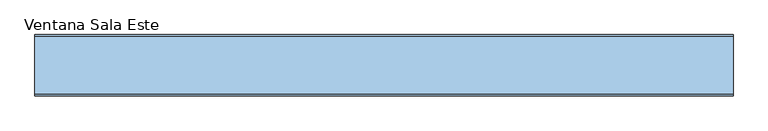
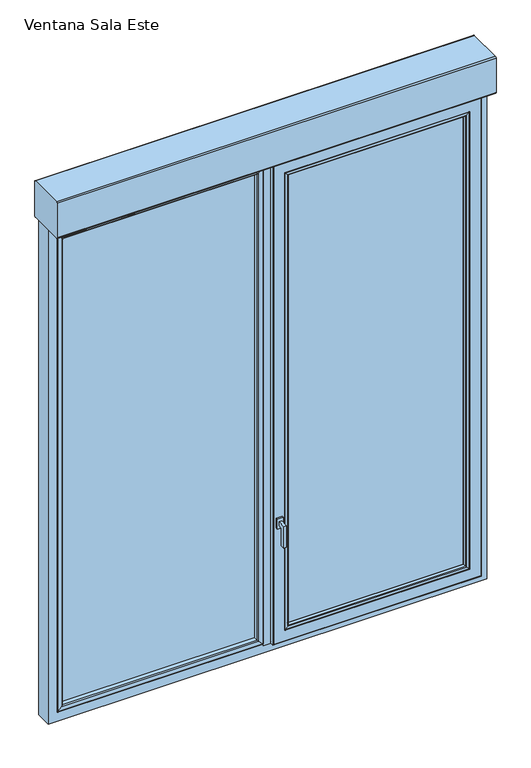
"""IFC4 building model written with IfcOpenShell, lengths in millimetres: window geometry, 2019_ES_Ventana_Replus_re80pvc301_11103_box_1-Hoja_Panel-Fijo-Lateral_con-Compacto : Ventana Sala Este."""

from ifc_helpers import new_model, si_unit, point, frame, frame_2d, origin, place, context, project, spatial, polyline, circle_curve, ellipse_curve, trimmed, segment, composite_curve, outline, extrude, source, transform, mapped, element, save
from ifc_brep_helpers import plane_surface, cylinder_surface, advanced_brep


def ventana_sala_este_de1b01aa(model_context):
    return source(origin(), model_context, "Body", "SolidModel", [
        extrude(outline(composite_curve([segment(polyline([(55.0, 3310.0), (-120.0, 3310.0)]), True, "CONTINUOUS"), segment(trimmed(circle_curve(frame_2d((-120.0, 3315.0)), 5.0), [point((-120.0, 3310.0))], [point((-125.0, 3315.0))], False, "CARTESIAN"), True, "CONTINUOUS"), segment(polyline([(-125.0, 3315.0), (-125.0, 3490.0)]), True, "CONTINUOUS"), segment(trimmed(circle_curve(frame_2d((-120.0, 3490.0)), 5.0), [point((-125.0, 3490.0))], [point((-120.0, 3495.0))], False, "CARTESIAN"), True, "CONTINUOUS"), segment(polyline([(-120.0, 3495.0), (55.0, 3495.0)]), True, "CONTINUOUS"), segment(trimmed(circle_curve(frame_2d((55.0, 3490.0)), 5.0), [point((55.0, 3495.0))], [point((60.0, 3490.0))], False, "CARTESIAN"), True, "CONTINUOUS"), segment(polyline([(60.0, 3490.0), (60.0, 3315.0)]), True, "CONTINUOUS"), segment(trimmed(circle_curve(frame_2d((55.0, 3315.0)), 5.0), [point((60.0, 3315.0))], [point((55.0, 3310.0))], False, "CARTESIAN"), True, "CONTINUOUS")], self_intersect=False)), frame((-1050.0, 0.0, 0.0), z_axis=(1.0, 0.0, 0.0), x_axis=(0.0, 1.0, 0.0)), (0.0, 0.0, 1.0), 2100.0),
        extrude(outline(polyline([(-78.4999991, 1470.0), (-78.4999991, 1450.0), (-98.4999991, 1450.0), (-98.4999991, 1360.0), (-118.4999991, 1360.0), (-118.4999991, 1470.0), (-78.4999991, 1470.0)])), frame((38.5, 0.0, 0.0), z_axis=(1.0, 0.0, 0.0), x_axis=(0.0, 1.0, 0.0)), (0.0, 0.0, 1.0), 12.0),
        extrude(outline(polyline([(58.7312385, -78.4999991), (30.2687615, -78.4999991), (30.2687615, -68.4999991), (58.7312385, -68.4999991), (58.7312385, -78.4999991)])), frame((0.0, 0.0, 1435.217127), z_axis=(0.0, 0.0, 1.0), x_axis=(1.0, 0.0, 0.0)), (0.0, 0.0, 1.0), 49.565746),
        extrude(outline(polyline([(-37.0063666, 11.4999962), (-37.0063666, 7.4999962), (-984.1891471, 7.4999962), (-984.1891471, 11.4999962), (-37.0063666, 11.4999962)])), frame((0.0, 0.0, 875.6108529), z_axis=(0.0, 0.0, 1.0), x_axis=(1.0, 0.0, 0.0)), (0.0, 0.0, 1.0), 2368.7782941),
        extrude(outline(polyline([(-37.0063666, -6.5), (-37.0063666, -10.5), (-984.1891471, -10.5), (-984.1891471, -6.5), (-37.0063666, -6.5)])), frame((0.0, 0.0, 875.6108529), z_axis=(0.0, 0.0, 1.0), x_axis=(1.0, 0.0, 0.0)), (0.0, 0.0, 1.0), 2368.7782941),
        extrude(outline(polyline([(-37.0063666, -24.4999997), (-37.0063666, -28.4999997), (-984.1891471, -28.4999997), (-984.1891471, -24.4999997), (-37.0063666, -24.4999997)])), frame((0.0, 0.0, 875.6108529), z_axis=(0.0, 0.0, 1.0), x_axis=(1.0, 0.0, 0.0)), (0.0, 0.0, 1.0), 2368.7782941),
        advanced_brep(
        [(-22.1502489, -49.9816666, 3264.0497511), (-41.8192398, -49.2838062, 3244.3807602), (-41.8192398, -49.2838062, 875.6192398), (-22.1502489, -49.9816666, 855.9502489), (-46.4697163, -45.5846502, 3239.7302837), (-46.4697163, -45.5846502, 880.2697163), (-984.3807594, -49.2838062, 875.6192398), (-1004.0497503, -49.9816666, 855.9502489), (-21.0, -48.871505, 3265.2), (-21.0, -48.871505, 854.8), (-51.0475336, -28.5000036, 3235.1524664), (-51.0475336, -28.5000036, 884.8475336), (-979.7302829, -45.5846502, 880.2697163), (-43.2922784, -28.5000036, 877.0922784), (-982.9077208, -28.5000036, 877.0922784), (-982.9077208, -28.5000036, 3242.9077216), (-43.2922784, -28.5000036, 3242.9077216), (-975.1524657, -28.5000036, 3235.1524664), (-975.1524657, -28.5000036, 884.8475336), (-35.4855, -36.306782, 3250.7145), (-35.4855, -36.306782, 869.2855), (-35.4855, -39.5069121, 3250.7145), (-35.4855, -39.5069121, 869.2855), (-990.7144993, -36.306782, 869.2855), (-21.0, -39.5069121, 854.8), (-1005.1999993, -39.5069121, 854.8), (-1005.1999993, -39.5069121, 3265.2), (-21.0, -39.5069121, 3265.2), (-990.7144993, -39.5069121, 3250.7145), (-990.7144993, -39.5069121, 869.2855), (-1005.1999993, -48.871505, 854.8), (-984.3807594, -49.2838062, 3244.3807602), (-1004.0497503, -49.9816666, 3264.0497511), (-979.7302829, -45.5846502, 3239.7302837), (-990.7144993, -36.306782, 3250.7145), (-1005.1999993, -48.871505, 3265.2)],
        [
            (0, 1),
            (1, 2),
            (2, 3),
            (3, 0),
            (1, 4, ellipse_curve(frame((-41.6449168, -44.2918491, 3244.5550832), z_axis=(0.7071067811865475, 0.0, -0.7071067811865475), x_axis=(0.7071067811865474, 0.0, 0.7071067811865476)), 7.0639967, 4.995)),
            (4, 5),
            (5, 2, ellipse_curve(frame((-41.6449168, -44.2918491, 875.4449168), z_axis=(0.7071067811865475, 0.0, 0.7071067811865475), x_axis=(-0.7071067811865474, 0.0, 0.7071067811865476)), 7.0639967, 4.995)),
            (2, 6),
            (6, 7),
            (7, 3),
            (8, 0, ellipse_curve(frame((-22.1108601, -48.871505, 3264.0891399), z_axis=(0.7071067811865475, 0.0, -0.7071067811865475), x_axis=(0.7071067811865474, 0.0, 0.7071067811865476)), 1.5709935, 1.1108601)),
            (3, 9, ellipse_curve(frame((-22.1108601, -48.871505, 855.9108601), z_axis=(0.7071067811865475, 0.0, 0.7071067811865475), x_axis=(-0.7071067811865474, 0.0, 0.7071067811865476)), 1.5709935, 1.1108601)),
            (9, 8),
            (4, 10),
            (10, 11),
            (11, 5),
            (5, 12),
            (12, 6, ellipse_curve(frame((-984.5550824, -44.2918491, 875.4449168), z_axis=(0.7071067811865475, 0.0, -0.7071067811865475), x_axis=(0.7071067811865476, 0.0, 0.7071067811865474)), 7.0639967, 4.995)),
            (13, 14),
            (14, 15),
            (15, 16),
            (16, 13),
            (10, 17),
            (17, 18),
            (18, 11),
            (18, 12),
            (16, 19),
            (19, 20),
            (20, 13),
            (19, 21),
            (21, 22),
            (22, 20),
            (20, 23),
            (23, 14),
            (24, 25),
            (25, 26),
            (26, 27),
            (27, 24),
            (21, 28),
            (28, 29),
            (29, 22),
            (29, 23),
            (9, 24),
            (27, 8),
            (9, 30),
            (30, 25),
            (7, 30, ellipse_curve(frame((-1004.0891391, -48.871505, 855.9108601), z_axis=(0.7071067811865475, 0.0, -0.7071067811865475), x_axis=(0.7071067811865476, 0.0, 0.7071067811865474)), 1.5709935, 1.1108601)),
            (6, 31),
            (31, 32),
            (32, 7),
            (12, 33),
            (33, 31, ellipse_curve(frame((-984.5550824, -44.2918491, 3244.5550832), z_axis=(-0.7071067811865475, 0.0, -0.7071067811865475), x_axis=(0.7071067811865474, 0.0, -0.7071067811865476)), 7.0639967, 4.995)),
            (17, 33),
            (23, 34),
            (34, 15),
            (28, 34),
            (30, 35),
            (35, 26),
            (32, 35, ellipse_curve(frame((-1004.0891391, -48.871505, 3264.0891399), z_axis=(-0.7071067811865475, 0.0, -0.7071067811865475), x_axis=(0.7071067811865474, 0.0, -0.7071067811865476)), 1.5709935, 1.1108601)),
            (31, 1),
            (0, 32),
            (33, 4),
            (34, 19),
            (35, 8),
        ],
        [
            plane_surface(frame((-41.8192398, -49.2838062, 3244.3807602), z_axis=(-0.03545791932093311, -0.9993711702652975, 0.0), x_axis=(0.0, 0.0, -1.0))),
            cylinder_surface(frame((-41.6449168, -44.2918491, 3272.2), z_axis=(0.0, 0.0, 1.0), x_axis=(-1.0, 0.0, 0.0)), 4.995),
            plane_surface(frame((-41.8192398, -49.2838062, 875.6192398), z_axis=(0.0, -0.9993711702652976, 0.035457919320929884), x_axis=(-1.0, 0.0, 0.0))),
            cylinder_surface(frame((-22.1108601, -48.871505, 3272.2), z_axis=(0.0, 0.0, 1.0), x_axis=(-1.0, 0.0, 0.0)), 1.1108601),
            plane_surface(frame((-51.0475336, -28.5000036, 3235.1524664), z_axis=(-0.9659258262890619, -0.25881904510254483, 0.0), x_axis=(0.0, 0.0, -1.0))),
            cylinder_surface(frame((-14.0, -44.2918491, 875.4449168), z_axis=(1.0, 0.0, 0.0), x_axis=(0.0, 0.0, 1.0)), 4.995),
            plane_surface(frame((-982.9077208, -28.5000036, 3242.9077216), z_axis=(0.0, 1.0, 0.0), x_axis=(1.0, 0.0, 0.0))),
            plane_surface(frame((-51.0475336, -28.5000036, 884.8475336), z_axis=(0.0, -0.25881904510254794, 0.965925826289061), x_axis=(-1.0, 0.0, 0.0))),
            plane_surface(frame((-35.4855, -36.306782, 3250.7145), z_axis=(0.7071067811865617, 0.7071067811865334, 0.0), x_axis=(0.0, 0.0, -1.0))),
            plane_surface(frame((-35.4855, -39.5069121, 3250.7145), z_axis=(1.0, 0.0, 0.0), x_axis=(0.0, 0.0, -1.0))),
            plane_surface(frame((-35.4855, -36.306782, 869.2855), z_axis=(0.0, 0.7071067811865357, -0.7071067811865593), x_axis=(-1.0, 0.0, 0.0))),
            plane_surface(frame((-1005.1999993, -39.5069121, 3265.2), z_axis=(0.0, 1.0, 0.0), x_axis=(1.0, 0.0, 0.0))),
            plane_surface(frame((-35.4855, -39.5069121, 869.2855), z_axis=(0.0, 0.0, -1.0), x_axis=(-1.0, 0.0, 0.0))),
            plane_surface(frame((-21.0, -46.2002121, 3265.2), z_axis=(1.0, 0.0, 0.0), x_axis=(0.0, 0.0, -1.0))),
            plane_surface(frame((-21.0, -46.2002121, 854.8), z_axis=(0.0, 0.0, -1.0), x_axis=(-1.0, 0.0, 0.0))),
            cylinder_surface(frame((-14.0, -48.871505, 855.9108601), z_axis=(1.0, 0.0, 0.0), x_axis=(0.0, 0.0, 1.0)), 1.1108601),
            plane_surface(frame((-984.3807594, -49.2838062, 875.6192398), z_axis=(0.03545791932092666, -0.9993711702652978, 0.0), x_axis=(0.0, 0.0, 1.0))),
            cylinder_surface(frame((-984.5550824, -44.2918491, 847.8), z_axis=(0.0, 0.0, -1.0), x_axis=(1.0, 0.0, 0.0)), 4.995),
            plane_surface(frame((-975.1524657, -28.5000036, 884.8475336), z_axis=(0.9659258262890602, -0.2588190451025511, 0.0), x_axis=(0.0, 0.0, 1.0))),
            plane_surface(frame((-990.7144993, -36.306782, 869.2855), z_axis=(-0.707106781186557, 0.707106781186538, 0.0), x_axis=(0.0, 0.0, 1.0))),
            plane_surface(frame((-990.7144993, -39.5069121, 869.2855), z_axis=(-1.0, 0.0, 0.0), x_axis=(0.0, 0.0, 1.0))),
            plane_surface(frame((-1005.1999993, -46.2002121, 854.8), z_axis=(-1.0, 0.0, 0.0), x_axis=(0.0, 0.0, 1.0))),
            cylinder_surface(frame((-1004.0891391, -48.871505, 847.8), z_axis=(0.0, 0.0, -1.0), x_axis=(1.0, 0.0, 0.0)), 1.1108601),
            plane_surface(frame((-984.3807594, -49.2838062, 3244.3807602), z_axis=(0.0, -0.9993711702652976, -0.035457919320929884), x_axis=(1.0, 0.0, 0.0))),
            cylinder_surface(frame((-1012.1999993, -44.2918491, 3244.5550832), z_axis=(-1.0, 0.0, 0.0), x_axis=(0.0, 0.0, -1.0)), 4.995),
            plane_surface(frame((-975.1524657, -28.5000036, 3235.1524664), z_axis=(0.0, -0.258819045102548, -0.9659258262890611), x_axis=(1.0, 0.0, 0.0))),
            plane_surface(frame((-990.7144993, -36.306782, 3250.7145), z_axis=(0.0, 0.7071067811865357, 0.7071067811865593), x_axis=(1.0, 0.0, 0.0))),
            plane_surface(frame((-990.7144993, -39.5069121, 3250.7145), z_axis=(0.0, 0.0, 1.0), x_axis=(1.0, 0.0, 0.0))),
            plane_surface(frame((-1005.1999993, -46.2002121, 3265.2), z_axis=(0.0, 0.0, 1.0), x_axis=(1.0, 0.0, 0.0))),
            cylinder_surface(frame((-1012.1999993, -48.871505, 3264.0891399), z_axis=(-1.0, 0.0, 0.0), x_axis=(0.0, 0.0, -1.0)), 1.1108601),
        ],
        [
            (0, [[1, 2, 3, 4]]),
            (1, [[5, 6, 7, -2]]),
            (2, [[-3, 8, 9, 10]]),
            (3, [[11, -4, 12, 13]]),
            (4, [[14, 15, 16, -6]]),
            (5, [[-7, 17, 18, -8]]),
            (6, [[19, 20, 21, 22], [23, 24, 25, -15]]),
            (7, [[-16, -25, 26, -17]]),
            (8, [[27, 28, 29, -22]]),
            (9, [[30, 31, 32, -28]]),
            (10, [[-29, 33, 34, -19]]),
            (11, [[35, 36, 37, 38], [39, 40, 41, -31]]),
            (12, [[-32, -41, 42, -33]]),
            (13, [[-13, 43, -38, 44]]),
            (14, [[-43, 45, 46, -35]]),
            (15, [[-12, -10, 47, -45]]),
            (16, [[-9, 48, 49, 50]]),
            (17, [[-18, 51, 52, -48]]),
            (18, [[-26, -24, 53, -51]]),
            (19, [[-34, 54, 55, -20]]),
            (20, [[-42, -40, 56, -54]]),
            (21, [[-46, 57, 58, -36]]),
            (22, [[-47, -50, 59, -57]]),
            (23, [[-49, 60, -1, 61]]),
            (24, [[-52, 62, -5, -60]]),
            (25, [[-53, -23, -14, -62]]),
            (26, [[-55, 63, -27, -21]]),
            (27, [[-56, -39, -30, -63]]),
            (28, [[-58, 64, -44, -37]]),
            (29, [[-59, -61, -11, -64]]),
        ],
    ),
        extrude(outline(polyline([(3207.0, 947.1999993), (3207.0, 81.0), (912.8, 81.0), (912.8, 947.1999993), (3207.0, 947.1999993)]), holes=[polyline([(920.8, 939.1999993), (920.8, 89.0), (3199.0, 89.0), (3199.0, 939.1999993), (920.8, 939.1999993)])]), frame((0.0, -27.0000002, 0.0), z_axis=(0.0, 1.0, 0.0), x_axis=(0.0, 0.0, 1.0)), (0.0, 0.0, 1.0), 16.0000002),
        extrude(outline(polyline([(3207.0, 947.1999993), (3207.0, 81.0), (912.8, 81.0), (912.8, 947.1999993), (3207.0, 947.1999993)]), holes=[polyline([(920.8, 939.1999993), (920.8, 89.0), (3199.0, 89.0), (3199.0, 939.1999993), (920.8, 939.1999993)])]), frame((0.0, -47.0000002, 0.0), z_axis=(0.0, 1.0, 0.0), x_axis=(0.0, 0.0, 1.0)), (0.0, 0.0, 1.0), 16.0000002),
        extrude(outline(polyline([(3238.3891471, -43.0063666), (3238.3891471, -978.1891471), (881.8608529, -978.1891471), (881.8608529, -43.0063666), (3238.3891471, -43.0063666)]), holes=[polyline([(889.8608529, -51.0063666), (889.8608529, -970.1891471), (3230.3891471, -970.1891471), (3230.3891471, -51.0063666), (889.8608529, -51.0063666)])]), frame((0.0, -24.5, 0.0), z_axis=(0.0, 1.0, 0.0), x_axis=(0.0, 0.0, 1.0)), (0.0, 0.0, 1.0), 14.0),
        extrude(outline(polyline([(3238.3891471, -43.0063666), (3238.3891471, -978.1891471), (881.8608529, -978.1891471), (881.8608529, -43.0063666), (3238.3891471, -43.0063666)]), holes=[polyline([(889.8608529, -51.0063666), (889.8608529, -970.1891471), (3230.3891471, -970.1891471), (3230.3891471, -51.0063666), (889.8608529, -51.0063666)])]), frame((0.0, -6.5, 0.0), z_axis=(0.0, 1.0, 0.0), x_axis=(0.0, 0.0, 1.0)), (0.0, 0.0, 1.0), 14.0),
        advanced_brep(
        [(48.1911809, 11.5, 3240.2), (48.1911809, 11.5, 879.8), (48.1911809, -11.9999991, 879.8), (48.1911809, -11.9999991, 3240.2), (980.1999993, 11.5, 3240.2), (980.1999993, 11.5, 879.8), (88.2020856, 11.5, 919.8109047), (940.1890945, 11.5, 919.8109047), (940.1890945, 11.5, 3200.1890953), (88.2020856, 11.5, 3200.1890953), (980.1999993, -11.9999991, 879.8), (35.1911809, -11.9999991, 3253.2), (993.1999993, -11.9999991, 3253.2), (993.1999993, -11.9999991, 866.8), (35.1911809, -11.9999991, 866.8), (980.1999993, -11.9999991, 3240.2), (35.1911809, -50.0, 866.8), (35.1911809, -50.0, 3253.2), (993.1999993, -50.0, 866.8), (15.1911809, -50.0, 3273.2), (1013.1999993, -50.0, 3273.2), (1013.1999993, -50.0, 846.8), (15.1911809, -50.0, 846.8), (993.1999993, -50.0, 3253.2), (15.1911809, -65.4999991, 3273.2), (15.1911809, -65.4999991, 846.8), (1013.1999993, -65.4999991, 846.8), (18.1911809, -68.4999991, 3270.2), (18.1911809, -68.4999991, 849.8), (1010.1999993, -68.4999991, 849.8), (1010.1999993, -68.4999991, 3270.2), (70.9541209, -68.4999991, 3217.43706), (957.4370593, -68.4999991, 3217.43706), (957.4370593, -68.4999991, 902.56294), (70.9541209, -68.4999991, 902.56294), (72.1911809, -67.2629391, 3216.2), (72.1911809, -67.2629391, 903.8), (956.1999993, -67.2629391, 903.8), (72.7423375, -67.7951848, 3215.6488434), (72.7423375, -67.7951848, 904.3511566), (955.6488427, -67.7951848, 904.3511566), (85.7676831, -67.3403297, 3202.6234978), (85.7676831, -67.3403297, 917.3765022), (942.6234971, -67.3403297, 917.3765022), (89.4917884, -64.3780426, 3198.8993925), (89.4917884, -64.3780426, 921.1006075), (938.8993918, -64.3780426, 921.1006075), (92.8970803, -51.6693201, 3195.4941006), (92.8970803, -51.6693201, 924.5058994), (935.4940999, -51.6693201, 924.5058994), (92.3834932, -51.0000003, 3196.0076877), (92.3834932, -51.0000003, 923.9923123), (936.007687, -51.0000003, 923.9923123), (81.1911809, -51.0000003, 3207.2), (947.1999993, -51.0000003, 3207.2), (947.1999993, -51.0000003, 912.8), (81.1911809, -51.0000003, 912.8), (936.007687, -51.0000003, 3196.0076877), (81.1911809, -56.4999995, 3207.2), (81.1911809, -56.4999995, 912.8), (947.1999993, -56.4999995, 912.8), (69.1911809, -56.4999995, 3219.2), (959.1999993, -56.4999995, 3219.2), (959.1999993, -56.4999995, 900.8), (69.1911809, -56.4999995, 900.8), (947.1999993, -56.4999995, 3207.2), (69.1911809, -25.6153717, 3219.2), (69.1911809, -25.6153717, 900.8), (959.1999993, -25.6153717, 900.8), (66.574961, -6.9999997, 3221.8162199), (66.574961, -6.9999997, 898.1837801), (961.8162192, -6.9999997, 898.1837801), (961.8162192, -6.9999997, 3221.8162199), (87.1911809, -6.9999997, 3201.2), (941.1999993, -6.9999997, 3201.2), (941.1999993, -6.9999997, 918.8), (87.1911809, -6.9999997, 918.8), (87.1911809, -3.0000033, 3201.2), (87.1911809, -3.0000033, 918.8), (941.1999993, -3.0000033, 918.8), (941.1999993, -3.0000033, 3201.2), (93.7172496, -3.0000033, 3194.6739313), (934.6739305, -3.0000033, 3194.6739313), (934.6739305, -3.0000033, 925.3260687), (93.7172496, -3.0000033, 925.3260687), (94.2153834, -2.3508228, 3194.1757976), (94.2153834, -2.3508228, 925.8242024), (934.1757968, -2.3508228, 925.8242024), (91.0998631, 9.2764571, 3197.2913178), (91.0998631, 9.2764571, 922.7086822), (937.2913171, 9.2764571, 922.7086822), (1013.1999993, -65.4999991, 3273.2), (956.1999993, -67.2629391, 3216.2), (955.6488427, -67.7951848, 3215.6488434), (942.6234971, -67.3403297, 3202.6234978), (938.8993918, -64.3780426, 3198.8993925), (935.4940999, -51.6693201, 3195.4941006), (959.1999993, -25.6153717, 3219.2), (934.1757968, -2.3508228, 3194.1757976), (937.2913171, 9.2764571, 3197.2913178)],
        [
            (0, 1),
            (1, 2),
            (2, 3),
            (3, 0),
            (0, 4),
            (4, 5),
            (5, 1),
            (6, 7),
            (7, 8),
            (8, 9),
            (9, 6),
            (5, 10),
            (10, 2),
            (11, 12),
            (12, 13),
            (13, 14),
            (14, 11),
            (10, 15),
            (15, 3),
            (14, 16),
            (16, 17),
            (17, 11),
            (13, 18),
            (18, 16),
            (19, 20),
            (20, 21),
            (21, 22),
            (22, 19),
            (18, 23),
            (23, 17),
            (24, 19),
            (22, 25),
            (25, 24),
            (21, 26),
            (26, 25),
            (27, 24, ellipse_curve(frame((18.1911809, -65.4999991, 3270.2), z_axis=(-0.7071067811865475, 0.0, -0.7071067811865475), x_axis=(-0.7071067811865474, 0.0, 0.7071067811865476)), 4.2426407, 3.0)),
            (25, 28, ellipse_curve(frame((18.1911809, -65.4999991, 849.8), z_axis=(-0.7071067811865475, 0.0, 0.7071067811865475), x_axis=(0.7071067811865474, 0.0, 0.7071067811865476)), 4.2426407, 3.0)),
            (28, 27),
            (26, 29, ellipse_curve(frame((1010.1999993, -65.4999991, 849.8), z_axis=(-0.7071067811865475, 0.0, -0.7071067811865475), x_axis=(-0.7071067811865476, 0.0, 0.7071067811865474)), 4.2426407, 3.0)),
            (29, 28),
            (29, 30),
            (30, 27),
            (31, 32),
            (32, 33),
            (33, 34),
            (34, 31),
            (35, 31, ellipse_curve(frame((70.9541209, -67.2629391, 3217.43706), z_axis=(-0.7071067811865475, 0.0, -0.7071067811865475), x_axis=(-0.7071067811865474, 0.0, 0.7071067811865476)), 1.7494671, 1.23706)),
            (34, 36, ellipse_curve(frame((70.9541209, -67.2629391, 902.56294), z_axis=(-0.7071067811865475, 0.0, 0.7071067811865475), x_axis=(0.7071067811865474, 0.0, 0.7071067811865476)), 1.7494671, 1.23706)),
            (36, 35),
            (33, 37, ellipse_curve(frame((957.4370593, -67.2629391, 902.56294), z_axis=(-0.7071067811865475, 0.0, -0.7071067811865475), x_axis=(-0.7071067811865476, 0.0, 0.7071067811865474)), 1.7494671, 1.23706)),
            (37, 36),
            (38, 35, ellipse_curve(frame((72.7237511, -67.2629391, 3215.6674299), z_axis=(-0.7071067811865475, 0.0, -0.7071067811865475), x_axis=(-0.7071067811865474, 0.0, 0.7071067811865476)), 0.7531679, 0.5325701)),
            (36, 39, ellipse_curve(frame((72.7237511, -67.2629391, 904.3325701), z_axis=(-0.7071067811865475, 0.0, 0.7071067811865475), x_axis=(0.7071067811865474, 0.0, 0.7071067811865476)), 0.7531679, 0.5325701)),
            (39, 38),
            (37, 40, ellipse_curve(frame((955.6674291, -67.2629391, 904.3325701), z_axis=(-0.7071067811865475, 0.0, -0.7071067811865475), x_axis=(-0.7071067811865476, 0.0, 0.7071067811865474)), 0.7531679, 0.5325701)),
            (40, 39),
            (41, 38),
            (39, 42),
            (42, 41),
            (40, 43),
            (43, 42),
            (44, 41, ellipse_curve(frame((85.6280851, -63.3427664, 3202.7630958), z_axis=(-0.7071067811865475, 0.0, -0.7071067811865475), x_axis=(-0.7071067811865474, 0.0, 0.7071067811865476)), 5.6568542, 4.0)),
            (42, 45, ellipse_curve(frame((85.6280851, -63.3427664, 917.2369042), z_axis=(-0.7071067811865475, 0.0, 0.7071067811865475), x_axis=(0.7071067811865474, 0.0, 0.7071067811865476)), 5.6568542, 4.0)),
            (45, 44),
            (43, 46, ellipse_curve(frame((942.7630951, -63.3427664, 917.2369042), z_axis=(-0.7071067811865475, 0.0, -0.7071067811865475), x_axis=(-0.7071067811865476, 0.0, 0.7071067811865474)), 5.6568542, 4.0)),
            (46, 45),
            (47, 44),
            (45, 48),
            (48, 47),
            (46, 49),
            (49, 48),
            (50, 47, ellipse_curve(frame((92.3834932, -51.5317048, 3196.0076877), z_axis=(-0.7071067811865475, 0.0, -0.7071067811865475), x_axis=(-0.7071067811865474, 0.0, 0.7071067811865476)), 0.7519437, 0.5317045)),
            (48, 51, ellipse_curve(frame((92.3834932, -51.5317048, 923.9923123), z_axis=(-0.7071067811865475, 0.0, 0.7071067811865475), x_axis=(0.7071067811865474, 0.0, 0.7071067811865476)), 0.7519437, 0.5317045)),
            (51, 50),
            (49, 52, ellipse_curve(frame((936.007687, -51.5317048, 923.9923123), z_axis=(-0.7071067811865475, 0.0, -0.7071067811865475), x_axis=(-0.7071067811865476, 0.0, 0.7071067811865474)), 0.7519437, 0.5317045)),
            (52, 51),
            (53, 54),
            (54, 55),
            (55, 56),
            (56, 53),
            (52, 57),
            (57, 50),
            (58, 53),
            (56, 59),
            (59, 58),
            (55, 60),
            (60, 59),
            (61, 62),
            (62, 63),
            (63, 64),
            (64, 61),
            (60, 65),
            (65, 58),
            (66, 61),
            (64, 67),
            (67, 66),
            (63, 68),
            (68, 67),
            (69, 66),
            (67, 70),
            (70, 69),
            (68, 71),
            (71, 70),
            (71, 72),
            (72, 69),
            (73, 74),
            (74, 75),
            (75, 76),
            (76, 73),
            (77, 73),
            (76, 78),
            (78, 77),
            (75, 79),
            (79, 78),
            (79, 80),
            (80, 77),
            (81, 82),
            (82, 83),
            (83, 84),
            (84, 81),
            (85, 81, ellipse_curve(frame((93.7172496, -2.4842973, 3194.6739313), z_axis=(-0.7071067811865475, 0.0, -0.7071067811865475), x_axis=(-0.7071067811865474, 0.0, 0.7071067811865476)), 0.7293184, 0.515706)),
            (84, 86, ellipse_curve(frame((93.7172496, -2.4842973, 925.3260687), z_axis=(-0.7071067811865475, 0.0, 0.7071067811865475), x_axis=(0.7071067811865474, 0.0, 0.7071067811865476)), 0.7293184, 0.515706)),
            (86, 85),
            (83, 87, ellipse_curve(frame((934.6739305, -2.4842973, 925.3260687), z_axis=(-0.7071067811865475, 0.0, -0.7071067811865475), x_axis=(-0.7071067811865476, 0.0, 0.7071067811865474)), 0.7293184, 0.515706)),
            (87, 86),
            (88, 85),
            (86, 89),
            (89, 88),
            (87, 90),
            (90, 89),
            (9, 88, ellipse_curve(frame((88.2020856, 8.5, 3200.1890953), z_axis=(-0.7071067811865475, 0.0, -0.7071067811865475), x_axis=(-0.7071067811865474, 0.0, 0.7071067811865476)), 4.2426407, 3.0)),
            (89, 6, ellipse_curve(frame((88.2020856, 8.5, 919.8109047), z_axis=(-0.7071067811865475, 0.0, 0.7071067811865475), x_axis=(0.7071067811865474, 0.0, 0.7071067811865476)), 4.2426407, 3.0)),
            (90, 7, ellipse_curve(frame((940.1890945, 8.5, 919.8109047), z_axis=(-0.7071067811865475, 0.0, -0.7071067811865475), x_axis=(-0.7071067811865476, 0.0, 0.7071067811865474)), 4.2426407, 3.0)),
            (4, 15),
            (12, 23),
            (20, 91),
            (91, 26),
            (91, 30, ellipse_curve(frame((1010.1999993, -65.4999991, 3270.2), z_axis=(0.7071067811865475, 0.0, -0.7071067811865475), x_axis=(-0.7071067811865474, 0.0, -0.7071067811865476)), 4.2426407, 3.0)),
            (32, 92, ellipse_curve(frame((957.4370593, -67.2629391, 3217.43706), z_axis=(0.7071067811865475, 0.0, -0.7071067811865475), x_axis=(-0.7071067811865474, 0.0, -0.7071067811865476)), 1.7494671, 1.23706)),
            (92, 37),
            (92, 93, ellipse_curve(frame((955.6674291, -67.2629391, 3215.6674299), z_axis=(0.7071067811865475, 0.0, -0.7071067811865475), x_axis=(-0.7071067811865474, 0.0, -0.7071067811865476)), 0.7531679, 0.5325701)),
            (93, 40),
            (93, 94),
            (94, 43),
            (94, 95, ellipse_curve(frame((942.7630951, -63.3427664, 3202.7630958), z_axis=(0.7071067811865475, 0.0, -0.7071067811865475), x_axis=(-0.7071067811865474, 0.0, -0.7071067811865476)), 5.6568542, 4.0)),
            (95, 46),
            (95, 96),
            (96, 49),
            (96, 57, ellipse_curve(frame((936.007687, -51.5317048, 3196.0076877), z_axis=(0.7071067811865475, 0.0, -0.7071067811865475), x_axis=(-0.7071067811865474, 0.0, -0.7071067811865476)), 0.7519437, 0.5317045)),
            (54, 65),
            (62, 97),
            (97, 68),
            (97, 72),
            (74, 80),
            (82, 98, ellipse_curve(frame((934.6739305, -2.4842973, 3194.6739313), z_axis=(0.7071067811865475, 0.0, -0.7071067811865475), x_axis=(-0.7071067811865474, 0.0, -0.7071067811865476)), 0.7293184, 0.515706)),
            (98, 87),
            (98, 99),
            (99, 90),
            (99, 8, ellipse_curve(frame((940.1890945, 8.5, 3200.1890953), z_axis=(0.7071067811865475, 0.0, -0.7071067811865475), x_axis=(-0.7071067811865474, 0.0, -0.7071067811865476)), 4.2426407, 3.0)),
            (24, 91),
            (35, 92),
            (38, 93),
            (41, 94),
            (44, 95),
            (47, 96),
            (66, 97),
            (85, 98),
            (88, 99),
        ],
        [
            plane_surface(frame((48.1911809, -1.4999991, 3240.2), z_axis=(-1.0, 0.0, 0.0), x_axis=(0.0, 0.0, -1.0))),
            plane_surface(frame((940.1890945, 11.5, 3200.1890953), z_axis=(0.0, 1.0, 0.0), x_axis=(-1.0, 0.0, 0.0))),
            plane_surface(frame((48.1911809, -1.4999991, 879.8), z_axis=(0.0, 0.0, -1.0), x_axis=(1.0, 0.0, 0.0))),
            plane_surface(frame((985.7000002, -11.9999991, 3245.7000009), z_axis=(0.0, 1.0, 0.0), x_axis=(-1.0, 0.0, 0.0))),
            plane_surface(frame((35.1911809, -45.0999991, 3253.2), z_axis=(-1.0, 0.0, 0.0), x_axis=(0.0, 0.0, -1.0))),
            plane_surface(frame((35.1911809, -45.0999991, 866.8), z_axis=(0.0, 0.0, -1.0), x_axis=(1.0, 0.0, 0.0))),
            plane_surface(frame((1009.2000019, -50.0, 3269.2000027), z_axis=(0.0, 1.0, 0.0), x_axis=(-1.0, 0.0, 0.0))),
            plane_surface(frame((15.1911809, -50.0, 3273.2), z_axis=(-1.0, 0.0, 0.0), x_axis=(0.0, 0.0, -1.0))),
            plane_surface(frame((15.1911809, -50.0, 846.8), z_axis=(0.0, 0.0, -1.0), x_axis=(1.0, 0.0, 0.0))),
            cylinder_surface(frame((18.1911809, -65.4999991, 3273.2), z_axis=(0.0, 0.0, 1.0), x_axis=(0.0, 1.0, 0.0)), 3.0),
            cylinder_surface(frame((15.1911809, -65.4999991, 849.8), z_axis=(-1.0, 0.0, 0.0), x_axis=(0.0, 1.0, 0.0)), 3.0),
            plane_surface(frame((1010.1999993, -68.4999991, 3270.2), z_axis=(0.0, -1.0, 0.0), x_axis=(-1.0, 0.0, 0.0))),
            cylinder_surface(frame((70.9541209, -67.2629391, 3273.2), z_axis=(0.0, 0.0, 1.0), x_axis=(0.0, 1.0, 0.0)), 1.23706),
            cylinder_surface(frame((15.1911809, -67.2629391, 902.56294), z_axis=(-1.0, 0.0, 0.0), x_axis=(0.0, 1.0, 0.0)), 1.23706),
            cylinder_surface(frame((72.7237511, -67.2629391, 3273.2), z_axis=(0.0, 0.0, 1.0), x_axis=(0.0, 1.0, 0.0)), 0.5325701),
            cylinder_surface(frame((15.1911809, -67.2629391, 904.3325701), z_axis=(-1.0, 0.0, 0.0), x_axis=(0.0, 1.0, 0.0)), 0.5325701),
            plane_surface(frame((72.7423375, -67.7951848, 3215.6488434), z_axis=(0.03489949670249966, -0.9993908270190959, 0.0), x_axis=(0.0, 0.0, -1.0))),
            plane_surface(frame((72.7423375, -67.7951848, 904.3511566), z_axis=(0.0, -0.9993908270190958, 0.034899496702502884), x_axis=(1.0, 0.0, 0.0))),
            cylinder_surface(frame((85.6280851, -63.3427664, 3273.2), z_axis=(0.0, 0.0, 1.0), x_axis=(0.0, 1.0, 0.0)), 4.0),
            cylinder_surface(frame((15.1911809, -63.3427664, 917.2369042), z_axis=(-1.0, 0.0, 0.0), x_axis=(0.0, 1.0, 0.0)), 4.0),
            plane_surface(frame((89.4917884, -64.3780426, 3198.8993925), z_axis=(0.9659258262890643, -0.2588190451025359, 0.0), x_axis=(0.0, 0.0, -1.0))),
            plane_surface(frame((89.4917884, -64.3780426, 921.1006075), z_axis=(0.0, -0.2588190451025328, 0.9659258262890652), x_axis=(1.0, 0.0, 0.0))),
            cylinder_surface(frame((92.3834932, -51.5317048, 3273.2), z_axis=(0.0, 0.0, 1.0), x_axis=(0.0, 1.0, 0.0)), 0.5317045),
            cylinder_surface(frame((15.1911809, -51.5317048, 923.9923123), z_axis=(-1.0, 0.0, 0.0), x_axis=(0.0, 1.0, 0.0)), 0.5317045),
            plane_surface(frame((936.007687, -51.0000003, 3196.0076877), z_axis=(0.0, 1.0, 0.0), x_axis=(-1.0, 0.0, 0.0))),
            plane_surface(frame((81.1911809, -51.0000003, 3207.2), z_axis=(-1.0, 0.0, 0.0), x_axis=(0.0, 0.0, -1.0))),
            plane_surface(frame((81.1911809, -51.0000003, 912.8), z_axis=(0.0, 0.0, -1.0), x_axis=(1.0, 0.0, 0.0))),
            plane_surface(frame((947.1999993, -56.4999995, 3207.2), z_axis=(0.0, 1.0, 0.0), x_axis=(-1.0, 0.0, 0.0))),
            plane_surface(frame((69.1911809, -56.4999995, 3219.2), z_axis=(1.0, 0.0, 0.0), x_axis=(0.0, 0.0, -1.0))),
            plane_surface(frame((69.1911809, -56.4999995, 900.8), z_axis=(0.0, 0.0, 1.0), x_axis=(1.0, 0.0, 0.0))),
            plane_surface(frame((69.1911809, -25.6153717, 3219.2), z_axis=(0.9902680687415736, 0.13917310096004257, 0.0), x_axis=(0.0, 0.0, -1.0))),
            plane_surface(frame((69.1911809, -25.6153717, 900.8), z_axis=(0.0, 0.13917310096004576, 0.9902680687415731), x_axis=(1.0, 0.0, 0.0))),
            plane_surface(frame((961.8162192, -6.9999997, 3221.8162199), z_axis=(0.0, -1.0, 0.0), x_axis=(-1.0, 0.0, 0.0))),
            plane_surface(frame((87.1911809, -6.9999997, 3201.2), z_axis=(1.0, 0.0, 0.0), x_axis=(0.0, 0.0, -1.0))),
            plane_surface(frame((87.1911809, -6.9999997, 918.8), z_axis=(0.0, 0.0, 1.0), x_axis=(1.0, 0.0, 0.0))),
            plane_surface(frame((941.1999993, -3.0000033, 3201.2), z_axis=(0.0, -1.0, 0.0), x_axis=(-1.0, 0.0, 0.0))),
            cylinder_surface(frame((93.7172496, -2.4842973, 3273.2), z_axis=(0.0, 0.0, 1.0), x_axis=(0.0, 1.0, 0.0)), 0.515706),
            cylinder_surface(frame((15.1911809, -2.4842973, 925.3260687), z_axis=(-1.0, 0.0, 0.0), x_axis=(0.0, 1.0, 0.0)), 0.515706),
            plane_surface(frame((94.2153834, -2.3508228, 3194.1757976), z_axis=(0.9659258263570589, 0.2588190448487762, 0.0), x_axis=(0.0, 0.0, -1.0))),
            plane_surface(frame((94.2153834, -2.3508228, 925.8242024), z_axis=(0.0, 0.2588190448487794, 0.9659258263570581), x_axis=(1.0, 0.0, 0.0))),
            cylinder_surface(frame((88.2020856, 8.5, 3273.2), z_axis=(0.0, 0.0, 1.0), x_axis=(0.0, 1.0, 0.0)), 3.0),
            cylinder_surface(frame((15.1911809, 8.5, 919.8109047), z_axis=(-1.0, 0.0, 0.0), x_axis=(0.0, 1.0, 0.0)), 3.0),
            plane_surface(frame((980.1999993, -1.4999991, 879.8), z_axis=(1.0, 0.0, 0.0), x_axis=(0.0, 0.0, 1.0))),
            plane_surface(frame((993.1999993, -45.0999991, 866.8), z_axis=(1.0, 0.0, 0.0), x_axis=(0.0, 0.0, 1.0))),
            plane_surface(frame((1013.1999993, -50.0, 846.8), z_axis=(1.0, 0.0, 0.0), x_axis=(0.0, 0.0, 1.0))),
            cylinder_surface(frame((1010.1999993, -65.4999991, 846.8), z_axis=(0.0, 0.0, -1.0), x_axis=(0.0, 1.0, 0.0)), 3.0),
            cylinder_surface(frame((957.4370593, -67.2629391, 846.8), z_axis=(0.0, 0.0, -1.0), x_axis=(0.0, 1.0, 0.0)), 1.23706),
            cylinder_surface(frame((955.6674291, -67.2629391, 846.8), z_axis=(0.0, 0.0, -1.0), x_axis=(0.0, 1.0, 0.0)), 0.5325701),
            plane_surface(frame((955.6488427, -67.7951848, 904.3511566), z_axis=(-0.03489949670250611, -0.9993908270190957, 0.0), x_axis=(0.0, 0.0, 1.0))),
            cylinder_surface(frame((942.7630951, -63.3427664, 846.8), z_axis=(0.0, 0.0, -1.0), x_axis=(0.0, 1.0, 0.0)), 4.0),
            plane_surface(frame((938.8993918, -64.3780426, 921.1006075), z_axis=(-0.965925826289066, -0.2588190451025297, 0.0), x_axis=(0.0, 0.0, 1.0))),
            cylinder_surface(frame((936.007687, -51.5317048, 846.8), z_axis=(0.0, 0.0, -1.0), x_axis=(0.0, 1.0, 0.0)), 0.5317045),
            plane_surface(frame((947.1999993, -51.0000003, 912.8), z_axis=(1.0, 0.0, 0.0), x_axis=(0.0, 0.0, 1.0))),
            plane_surface(frame((959.1999993, -56.4999995, 900.8), z_axis=(-1.0, 0.0, 0.0), x_axis=(0.0, 0.0, 1.0))),
            plane_surface(frame((959.1999993, -25.6153717, 900.8), z_axis=(-0.9902680687415727, 0.13917310096004895, 0.0), x_axis=(0.0, 0.0, 1.0))),
            plane_surface(frame((941.1999993, -6.9999997, 918.8), z_axis=(-1.0, 0.0, 0.0), x_axis=(0.0, 0.0, 1.0))),
            cylinder_surface(frame((934.6739305, -2.4842973, 846.8), z_axis=(0.0, 0.0, -1.0), x_axis=(0.0, 1.0, 0.0)), 0.515706),
            plane_surface(frame((934.1757968, -2.3508228, 925.8242024), z_axis=(-0.9659258263570573, 0.2588190448487825, 0.0), x_axis=(0.0, 0.0, 1.0))),
            cylinder_surface(frame((940.1890945, 8.5, 846.8), z_axis=(0.0, 0.0, -1.0), x_axis=(0.0, 1.0, 0.0)), 3.0),
            plane_surface(frame((980.1999993, -1.4999991, 3240.2), z_axis=(0.0, 0.0, 1.0), x_axis=(-1.0, 0.0, 0.0))),
            plane_surface(frame((993.1999993, -45.0999991, 3253.2), z_axis=(0.0, 0.0, 1.0), x_axis=(-1.0, 0.0, 0.0))),
            plane_surface(frame((1013.1999993, -50.0, 3273.2), z_axis=(0.0, 0.0, 1.0), x_axis=(-1.0, 0.0, 0.0))),
            cylinder_surface(frame((1013.1999993, -65.4999991, 3270.2), z_axis=(1.0, 0.0, 0.0), x_axis=(0.0, 1.0, 0.0)), 3.0),
            cylinder_surface(frame((1013.1999993, -67.2629391, 3217.43706), z_axis=(1.0, 0.0, 0.0), x_axis=(0.0, 1.0, 0.0)), 1.23706),
            cylinder_surface(frame((1013.1999993, -67.2629391, 3215.6674299), z_axis=(1.0, 0.0, 0.0), x_axis=(0.0, 1.0, 0.0)), 0.5325701),
            plane_surface(frame((955.6488427, -67.7951848, 3215.6488434), z_axis=(0.0, -0.9993908270190958, -0.034899496702502884), x_axis=(-1.0, 0.0, 0.0))),
            cylinder_surface(frame((1013.1999993, -63.3427664, 3202.7630958), z_axis=(1.0, 0.0, 0.0), x_axis=(0.0, 1.0, 0.0)), 4.0),
            plane_surface(frame((938.8993918, -64.3780426, 3198.8993925), z_axis=(0.0, -0.2588190451025328, -0.9659258262890651), x_axis=(-1.0, 0.0, 0.0))),
            cylinder_surface(frame((1013.1999993, -51.5317048, 3196.0076877), z_axis=(1.0, 0.0, 0.0), x_axis=(0.0, 1.0, 0.0)), 0.5317045),
            plane_surface(frame((947.1999993, -51.0000003, 3207.2), z_axis=(0.0, 0.0, 1.0), x_axis=(-1.0, 0.0, 0.0))),
            plane_surface(frame((959.1999993, -56.4999995, 3219.2), z_axis=(0.0, 0.0, -1.0), x_axis=(-1.0, 0.0, 0.0))),
            plane_surface(frame((959.1999993, -25.6153717, 3219.2), z_axis=(0.0, 0.13917310096004576, -0.9902680687415731), x_axis=(-1.0, 0.0, 0.0))),
            plane_surface(frame((941.1999993, -6.9999997, 3201.2), z_axis=(0.0, 0.0, -1.0), x_axis=(-1.0, 0.0, 0.0))),
            cylinder_surface(frame((1013.1999993, -2.4842973, 3194.6739313), z_axis=(1.0, 0.0, 0.0), x_axis=(0.0, 1.0, 0.0)), 0.515706),
            plane_surface(frame((934.1757968, -2.3508228, 3194.1757976), z_axis=(0.0, 0.2588190448487794, -0.9659258263570581), x_axis=(-1.0, 0.0, 0.0))),
            cylinder_surface(frame((1013.1999993, 8.5, 3200.1890953), z_axis=(1.0, 0.0, 0.0), x_axis=(0.0, 1.0, 0.0)), 3.0),
        ],
        [
            (0, [[1, 2, 3, 4]]),
            (1, [[5, 6, 7, -1], [8, 9, 10, 11]]),
            (2, [[-2, -7, 12, 13]]),
            (3, [[14, 15, 16, 17], [-13, 18, 19, -3]]),
            (4, [[-17, 20, 21, 22]]),
            (5, [[-20, -16, 23, 24]]),
            (6, [[25, 26, 27, 28], [-24, 29, 30, -21]]),
            (7, [[31, -28, 32, 33]]),
            (8, [[-32, -27, 34, 35]]),
            (9, [[36, -33, 37, 38]]),
            (10, [[-37, -35, 39, 40]]),
            (11, [[-40, 41, 42, -38], [43, 44, 45, 46]]),
            (12, [[47, -46, 48, 49]]),
            (13, [[-48, -45, 50, 51]]),
            (14, [[52, -49, 53, 54]]),
            (15, [[-53, -51, 55, 56]]),
            (16, [[57, -54, 58, 59]]),
            (17, [[-58, -56, 60, 61]]),
            (18, [[62, -59, 63, 64]]),
            (19, [[-63, -61, 65, 66]]),
            (20, [[67, -64, 68, 69]]),
            (21, [[-68, -66, 70, 71]]),
            (22, [[72, -69, 73, 74]]),
            (23, [[-73, -71, 75, 76]]),
            (24, [[77, 78, 79, 80], [-76, 81, 82, -74]]),
            (25, [[83, -80, 84, 85]]),
            (26, [[-84, -79, 86, 87]]),
            (27, [[88, 89, 90, 91], [-87, 92, 93, -85]]),
            (28, [[94, -91, 95, 96]]),
            (29, [[-95, -90, 97, 98]]),
            (30, [[99, -96, 100, 101]]),
            (31, [[-100, -98, 102, 103]]),
            (32, [[-103, 104, 105, -101], [106, 107, 108, 109]]),
            (33, [[110, -109, 111, 112]]),
            (34, [[-111, -108, 113, 114]]),
            (35, [[-114, 115, 116, -112], [117, 118, 119, 120]]),
            (36, [[121, -120, 122, 123]]),
            (37, [[-122, -119, 124, 125]]),
            (38, [[126, -123, 127, 128]]),
            (39, [[-127, -125, 129, 130]]),
            (40, [[131, -128, 132, -11]]),
            (41, [[-132, -130, 133, -8]]),
            (42, [[-12, -6, 134, -18]]),
            (43, [[-23, -15, 135, -29]]),
            (44, [[-34, -26, 136, 137]]),
            (45, [[-39, -137, 138, -41]]),
            (46, [[-50, -44, 139, 140]]),
            (47, [[-55, -140, 141, 142]]),
            (48, [[-60, -142, 143, 144]]),
            (49, [[-65, -144, 145, 146]]),
            (50, [[-70, -146, 147, 148]]),
            (51, [[-75, -148, 149, -81]]),
            (52, [[-86, -78, 150, -92]]),
            (53, [[-97, -89, 151, 152]]),
            (54, [[-102, -152, 153, -104]]),
            (55, [[-113, -107, 154, -115]]),
            (56, [[-124, -118, 155, 156]]),
            (57, [[-129, -156, 157, 158]]),
            (58, [[-133, -158, 159, -9]]),
            (59, [[-134, -5, -4, -19]]),
            (60, [[-135, -14, -22, -30]]),
            (61, [[-136, -25, -31, 160]]),
            (62, [[-138, -160, -36, -42]]),
            (63, [[-139, -43, -47, 161]]),
            (64, [[-141, -161, -52, 162]]),
            (65, [[-143, -162, -57, 163]]),
            (66, [[-145, -163, -62, 164]]),
            (67, [[-147, -164, -67, 165]]),
            (68, [[-149, -165, -72, -82]]),
            (69, [[-150, -77, -83, -93]]),
            (70, [[-151, -88, -94, 166]]),
            (71, [[-153, -166, -99, -105]]),
            (72, [[-154, -106, -110, -116]]),
            (73, [[-155, -117, -121, 167]]),
            (74, [[-157, -167, -126, 168]]),
            (75, [[-159, -168, -131, -10]]),
        ],
    ),
        extrude(outline(composite_curve([segment(polyline([(23.3911809, -37.9746327), (23.3911809, -49.0)]), True, "CONTINUOUS"), segment(trimmed(circle_curve(frame_2d((22.3911809, -49.0)), 1.0), [point((23.3911809, -49.0))], [point((22.3911809, -50.0))], False, "CARTESIAN"), True, "CONTINUOUS"), segment(polyline([(22.3911809, -50.0), (-19.7446784, -50.0)]), True, "CONTINUOUS"), segment(trimmed(circle_curve(frame_2d((-19.7446784, -49.0)), 1.0), [point((-19.7446784, -50.0))], [point((-20.7446784, -49.0))], False, "CARTESIAN"), True, "CONTINUOUS"), segment(polyline([(-20.7446784, -49.0), (-20.7446784, -37.9746327), (-18.5911809, -37.9746327), (-18.5911809, -8.0), (-40.6020331, -8.0), (-40.6020331, -6.2175904), (-27.9799071, 1.0697975), (-26.7556588, 15.0630198), (-41.0115567, 17.0665556), (-41.7938856, 11.4999962), (-52.5579009, 11.4999962)]), True, "CONTINUOUS"), segment(trimmed(circle_curve(frame_2d((-52.5579009, 12.4999962)), 1.0), [point((-52.5579009, 11.4999962))], [point((-53.5238267, 12.7588152))], False, "CARTESIAN"), True, "CONTINUOUS"), segment(polyline([(-53.5238267, 12.7588152), (-49.4998617, 27.7764571)]), True, "CONTINUOUS"), segment(trimmed(circle_curve(frame_2d((-46.6020842, 27.0)), 3.0), [point((-49.4998617, 27.7764571))], [point((-46.6020842, 30.0))], False, "CARTESIAN"), True, "CONTINUOUS"), segment(polyline([(-46.6020842, 30.0), (48.4020842, 30.0)]), True, "CONTINUOUS"), segment(trimmed(circle_curve(frame_2d((48.4020842, 27.0)), 3.0), [point((48.4020842, 30.0))], [point((51.2998617, 27.7764571))], False, "CARTESIAN"), True, "CONTINUOUS"), segment(polyline([(51.2998617, 27.7764571), (55.3238267, 12.7588152)]), True, "CONTINUOUS"), segment(trimmed(circle_curve(frame_2d((54.3579009, 12.4999962)), 1.0), [point((55.3238267, 12.7588152))], [point((54.3579009, 11.4999962))], False, "CARTESIAN"), True, "CONTINUOUS"), segment(polyline([(54.3579009, 11.4999962), (43.5938856, 11.4999962), (42.8115567, 17.0665556), (28.5556588, 15.0630198), (29.7799071, 1.0697975), (42.4020331, -6.2175904), (42.4020331, -8.0), (20.3911809, -8.0), (20.3911809, -37.9746327), (23.3911809, -37.9746327)]), True, "CONTINUOUS")], self_intersect=False)), frame((0.0, 0.0, 846.8), z_axis=(0.0, 0.0, 1.0), x_axis=(1.0, 0.0, 0.0)), (0.0, 0.0, 1.0), 2426.4),
        extrude(outline(polyline([(953.1999993, -6.9999997), (953.1999993, -10.9999997), (75.0, -10.9999997), (75.0, -6.9999997), (953.1999993, -6.9999997)])), frame((0.0, 0.0, 906.8), z_axis=(0.0, 0.0, 1.0), x_axis=(1.0, 0.0, 0.0)), (0.0, 0.0, 1.0), 2306.2),
        extrude(outline(polyline([(953.1999993, -26.9999997), (953.1999993, -30.9999997), (75.0, -30.9999997), (75.0, -26.9999997), (953.1999993, -26.9999997)])), frame((0.0, 0.0, 906.8), z_axis=(0.0, 0.0, 1.0), x_axis=(1.0, 0.0, 0.0)), (0.0, 0.0, 1.0), 2306.2),
        extrude(outline(polyline([(953.1999993, -46.9999997), (953.1999993, -50.9999997), (75.0, -50.9999997), (75.0, -46.9999997), (953.1999993, -46.9999997)])), frame((0.0, 0.0, 906.8), z_axis=(0.0, 0.0, 1.0), x_axis=(1.0, 0.0, 0.0)), (0.0, 0.0, 1.0), 2306.2),
        advanced_brep(
        [(1006.1999993, -50.0, 3266.1999993), (1005.1999993, -49.0, 3265.1999993), (1005.1999993, -49.0, 854.8000007), (1006.1999993, -50.0, 853.8000007), (1005.1999993, -8.0, 3265.1999993), (1005.1999993, -8.0, 854.8000007), (-1005.1999993, -49.0, 854.8000007), (-1006.1999993, -50.0, 853.8000007), (1050.0, -50.0, 3310.0), (-1050.0, -50.0, 3310.0), (-1050.0, -50.0, 810.0), (1050.0, -50.0, 810.0), (-1006.1999993, -50.0, 3266.1999993), (974.2332803, 11.5, 3234.2332803), (973.2673545, 12.758819, 3233.2673545), (973.2673545, 12.758819, 886.7326455), (974.2332803, 11.5, 885.7667197), (977.2913185, 27.7764571, 3237.2913185), (977.2913185, 27.7764571, 882.7086815), (-973.2673545, 12.758819, 886.7326455), (-974.2332803, 11.5, 885.7667197), (986.1891471, 11.5, 3246.1891471), (-986.1891471, 11.5, 3246.1891471), (-986.1891471, 11.5, 873.8108529), (986.1891471, 11.5, 873.8108529), (-974.2332803, 11.5, 3234.2332803), (980.189096, 30.0, 3240.189096), (980.189096, 30.0, 879.810904), (1050.0, 30.0, 810.0), (-1050.0, 30.0, 810.0), (-1050.0, 30.0, 3310.0), (1050.0, 30.0, 3310.0), (-980.189096, 30.0, 3240.189096), (-980.189096, 30.0, 879.810904), (-977.2913185, 27.7764571, 882.7086815), (986.1891471, -8.0, 3246.1891471), (986.1891471, -8.0, 873.8108529), (-986.1891471, -8.0, 873.8108529), (-1005.1999993, -8.0, 3265.1999993), (-1005.1999993, -8.0, 854.8000007), (-986.1891471, -8.0, 3246.1891471), (-1005.1999993, -49.0, 3265.1999993), (-973.2673545, 12.758819, 3233.2673545), (-977.2913185, 27.7764571, 3237.2913185)],
        [
            (0, 1, ellipse_curve(frame((1006.1999993, -49.0, 3266.1999993), z_axis=(0.7071067811865475, 0.0, -0.7071067811865475), x_axis=(0.7071067811865474, 0.0, 0.7071067811865476)), 1.4142136, 1.0)),
            (1, 2),
            (2, 3, ellipse_curve(frame((1006.1999993, -49.0, 853.8000007), z_axis=(0.7071067811865475, 0.0, 0.7071067811865475), x_axis=(-0.7071067811865474, 0.0, 0.7071067811865476)), 1.4142136, 1.0)),
            (3, 0),
            (1, 4),
            (4, 5),
            (5, 2),
            (2, 6),
            (6, 7, ellipse_curve(frame((-1006.1999993, -49.0, 853.8000007), z_axis=(0.7071067811865475, 0.0, -0.7071067811865475), x_axis=(0.7071067811865476, 0.0, 0.7071067811865474)), 1.4142136, 1.0)),
            (7, 3),
            (8, 9),
            (9, 10),
            (10, 11),
            (11, 8),
            (7, 12),
            (12, 0),
            (13, 14, ellipse_curve(frame((974.2332803, 12.5, 3234.2332803), z_axis=(0.7071067811865475, 0.0, -0.7071067811865475), x_axis=(0.7071067811865474, 0.0, 0.7071067811865476)), 1.4142136, 1.0)),
            (14, 15),
            (15, 16, ellipse_curve(frame((974.2332803, 12.5, 885.7667197), z_axis=(0.7071067811865475, 0.0, 0.7071067811865475), x_axis=(-0.7071067811865474, 0.0, 0.7071067811865476)), 1.4142136, 1.0)),
            (16, 13),
            (14, 17),
            (17, 18),
            (18, 15),
            (15, 19),
            (19, 20, ellipse_curve(frame((-974.2332803, 12.5, 885.7667197), z_axis=(0.7071067811865475, 0.0, -0.7071067811865475), x_axis=(0.7071067811865476, 0.0, 0.7071067811865474)), 1.4142136, 1.0)),
            (20, 16),
            (21, 22),
            (22, 23),
            (23, 24),
            (24, 21),
            (20, 25),
            (25, 13),
            (17, 26, ellipse_curve(frame((980.189096, 27.0, 3240.189096), z_axis=(0.7071067811865475, 0.0, -0.7071067811865475), x_axis=(0.7071067811865474, 0.0, 0.7071067811865476)), 4.2426407, 3.0)),
            (26, 27),
            (27, 18, ellipse_curve(frame((980.189096, 27.0, 879.810904), z_axis=(0.7071067811865475, 0.0, 0.7071067811865475), x_axis=(-0.7071067811865474, 0.0, 0.7071067811865476)), 4.2426407, 3.0)),
            (28, 29),
            (29, 30),
            (30, 31),
            (31, 28),
            (26, 32),
            (32, 33),
            (33, 27),
            (33, 34, ellipse_curve(frame((-980.189096, 27.0, 879.810904), z_axis=(0.7071067811865475, 0.0, -0.7071067811865475), x_axis=(0.7071067811865476, 0.0, 0.7071067811865474)), 4.2426407, 3.0)),
            (34, 18),
            (34, 19),
            (35, 21),
            (24, 36),
            (36, 35),
            (23, 37),
            (37, 36),
            (4, 38),
            (38, 39),
            (39, 5),
            (37, 40),
            (40, 35),
            (31, 8),
            (11, 28),
            (10, 29),
            (39, 6),
            (6, 41),
            (41, 12, ellipse_curve(frame((-1006.1999993, -49.0, 3266.1999993), z_axis=(-0.7071067811865475, 0.0, -0.7071067811865475), x_axis=(0.7071067811865474, 0.0, -0.7071067811865476)), 1.4142136, 1.0)),
            (19, 42),
            (42, 25, ellipse_curve(frame((-974.2332803, 12.5, 3234.2332803), z_axis=(-0.7071067811865475, 0.0, -0.7071067811865475), x_axis=(0.7071067811865474, 0.0, -0.7071067811865476)), 1.4142136, 1.0)),
            (32, 43, ellipse_curve(frame((-980.189096, 27.0, 3240.189096), z_axis=(-0.7071067811865475, 0.0, -0.7071067811865475), x_axis=(0.7071067811865474, 0.0, -0.7071067811865476)), 4.2426407, 3.0)),
            (43, 34),
            (43, 42),
            (22, 40),
            (9, 30),
            (38, 41),
            (41, 1),
            (42, 14),
            (17, 43),
        ],
        [
            cylinder_surface(frame((1006.1999993, -49.0, 3310.0), z_axis=(0.0, 0.0, 1.0), x_axis=(-1.0, 0.0, 0.0)), 1.0),
            plane_surface(frame((1005.1999993, -8.0, 3265.1999993), z_axis=(-1.0, 0.0, 0.0), x_axis=(0.0, 0.0, -1.0))),
            cylinder_surface(frame((1050.0, -49.0, 853.8000007), z_axis=(1.0, 0.0, 0.0), x_axis=(0.0, 0.0, 1.0)), 1.0),
            plane_surface(frame((-1006.1999993, -50.0, 3266.1999993), z_axis=(0.0, -1.0, 0.0), x_axis=(1.0, 0.0, 0.0))),
            cylinder_surface(frame((974.2332803, 12.5, 3310.0), z_axis=(0.0, 0.0, 1.0), x_axis=(-1.0, 0.0, 0.0)), 1.0),
            plane_surface(frame((977.2913185, 27.7764571, 3237.2913185), z_axis=(-0.9659258262890672, 0.25881904510252485, 0.0), x_axis=(0.0, 0.0, -1.0))),
            cylinder_surface(frame((1050.0, 12.5, 885.7667197), z_axis=(1.0, 0.0, 0.0), x_axis=(0.0, 0.0, 1.0)), 1.0),
            plane_surface(frame((-974.2332803, 11.5, 3234.2332803), z_axis=(0.0, -1.0, 0.0), x_axis=(1.0, 0.0, 0.0))),
            cylinder_surface(frame((980.189096, 27.0, 3310.0), z_axis=(0.0, 0.0, 1.0), x_axis=(-1.0, 0.0, 0.0)), 3.0),
            plane_surface(frame((-1050.0, 30.0, 3310.0), z_axis=(0.0, 1.0, 0.0), x_axis=(1.0, 0.0, 0.0))),
            cylinder_surface(frame((1050.0, 27.0, 879.810904), z_axis=(1.0, 0.0, 0.0), x_axis=(0.0, 0.0, 1.0)), 3.0),
            plane_surface(frame((977.2913185, 27.7764571, 882.7086815), z_axis=(0.0, 0.25881904510252174, 0.9659258262890681), x_axis=(-1.0, 0.0, 0.0))),
            plane_surface(frame((986.1891471, 11.5, 3246.1891471), z_axis=(-1.0, 0.0, 0.0), x_axis=(0.0, 0.0, -1.0))),
            plane_surface(frame((986.1891471, 11.5, 873.8108529), z_axis=(0.0, 0.0, 1.0), x_axis=(-1.0, 0.0, 0.0))),
            plane_surface(frame((-986.1891471, -8.0, 3246.1891471), z_axis=(0.0, -1.0, 0.0), x_axis=(1.0, 0.0, 0.0))),
            plane_surface(frame((1050.0, -50.0, 3310.0), z_axis=(1.0, 0.0, 0.0), x_axis=(0.0, 0.0, -1.0))),
            plane_surface(frame((1050.0, -50.0, 810.0), z_axis=(0.0, 0.0, -1.0), x_axis=(-1.0, 0.0, 0.0))),
            plane_surface(frame((1005.1999993, -8.0, 854.8000007), z_axis=(0.0, 0.0, 1.0), x_axis=(-1.0, 0.0, 0.0))),
            cylinder_surface(frame((-1006.1999993, -49.0, 810.0), z_axis=(0.0, 0.0, -1.0), x_axis=(1.0, 0.0, 0.0)), 1.0),
            cylinder_surface(frame((-974.2332803, 12.5, 810.0), z_axis=(0.0, 0.0, -1.0), x_axis=(1.0, 0.0, 0.0)), 1.0),
            cylinder_surface(frame((-980.189096, 27.0, 810.0), z_axis=(0.0, 0.0, -1.0), x_axis=(1.0, 0.0, 0.0)), 3.0),
            plane_surface(frame((-977.2913185, 27.7764571, 882.7086815), z_axis=(0.965925826289069, 0.25881904510251863, 0.0), x_axis=(0.0, 0.0, 1.0))),
            plane_surface(frame((-986.1891471, 11.5, 873.8108529), z_axis=(1.0, 0.0, 0.0), x_axis=(0.0, 0.0, 1.0))),
            plane_surface(frame((-1050.0, -50.0, 810.0), z_axis=(-1.0, 0.0, 0.0), x_axis=(0.0, 0.0, 1.0))),
            plane_surface(frame((-1005.1999993, -8.0, 854.8000007), z_axis=(1.0, 0.0, 0.0), x_axis=(0.0, 0.0, 1.0))),
            cylinder_surface(frame((-1050.0, -49.0, 3266.1999993), z_axis=(-1.0, 0.0, 0.0), x_axis=(0.0, 0.0, -1.0)), 1.0),
            cylinder_surface(frame((-1050.0, 12.5, 3234.2332803), z_axis=(-1.0, 0.0, 0.0), x_axis=(0.0, 0.0, -1.0)), 1.0),
            cylinder_surface(frame((-1050.0, 27.0, 3240.189096), z_axis=(-1.0, 0.0, 0.0), x_axis=(0.0, 0.0, -1.0)), 3.0),
            plane_surface(frame((-977.2913185, 27.7764571, 3237.2913185), z_axis=(0.0, 0.25881904510252174, -0.9659258262890681), x_axis=(1.0, 0.0, 0.0))),
            plane_surface(frame((-986.1891471, 11.5, 3246.1891471), z_axis=(0.0, 0.0, -1.0), x_axis=(1.0, 0.0, 0.0))),
            plane_surface(frame((-1050.0, -50.0, 3310.0), z_axis=(0.0, 0.0, 1.0), x_axis=(1.0, 0.0, 0.0))),
            plane_surface(frame((-1005.1999993, -8.0, 3265.1999993), z_axis=(0.0, 0.0, -1.0), x_axis=(1.0, 0.0, 0.0))),
        ],
        [
            (0, [[1, 2, 3, 4]]),
            (1, [[5, 6, 7, -2]]),
            (2, [[-3, 8, 9, 10]]),
            (3, [[11, 12, 13, 14], [-10, 15, 16, -4]]),
            (4, [[17, 18, 19, 20]]),
            (5, [[21, 22, 23, -18]]),
            (6, [[-19, 24, 25, 26]]),
            (7, [[27, 28, 29, 30], [-26, 31, 32, -20]]),
            (8, [[33, 34, 35, -22]]),
            (9, [[36, 37, 38, 39], [40, 41, 42, -34]]),
            (10, [[-35, -42, 43, 44]]),
            (11, [[-23, -44, 45, -24]]),
            (12, [[46, -30, 47, 48]]),
            (13, [[-47, -29, 49, 50]]),
            (14, [[51, 52, 53, -6], [-50, 54, 55, -48]]),
            (15, [[56, -14, 57, -39]]),
            (16, [[-57, -13, 58, -36]]),
            (17, [[-7, -53, 59, -8]]),
            (18, [[-9, 60, 61, -15]]),
            (19, [[-25, 62, 63, -31]]),
            (20, [[-43, -41, 64, 65]]),
            (21, [[-45, -65, 66, -62]]),
            (22, [[-49, -28, 67, -54]]),
            (23, [[-58, -12, 68, -37]]),
            (24, [[-59, -52, 69, -60]]),
            (25, [[-61, 70, -1, -16]]),
            (26, [[-63, 71, -17, -32]]),
            (27, [[-64, -40, -33, 72]]),
            (28, [[-66, -72, -21, -71]]),
            (29, [[-67, -27, -46, -55]]),
            (30, [[-68, -11, -56, -38]]),
            (31, [[-69, -51, -5, -70]]),
        ],
    ),
    ])


if __name__ == "__main__":
    model = new_model("IFC4")
    model_context = context("Model", 3, world=origin())
    ifc_project = project(units=[si_unit("LENGTHUNIT", "METRE", prefix="MILLI")], contexts=[model_context])
    site = spatial("IfcSite", under=ifc_project)
    building = spatial("IfcBuilding", under=site)
    placement = place(None, origin())
    ventana_sala_este_shape = ventana_sala_este_de1b01aa(model_context)
    element("IfcWindow", 1, ObjectType="2019_ES_Ventana_Replus_re80pvc301_11103_box_1-Hoja_Panel-Fijo-Lateral_con-Compacto : Ventana Sala Este", at=placement, inside=building, context=model_context, shape_type="MappedRepresentation", body=[
        mapped(ventana_sala_este_shape, transform((0.0, 0.0, 0.0), x_axis=(1.0, 0.0, 0.0), y_axis=(0.0, 1.0, 0.0), z_axis=(0.0, 0.0, 1.0))),
    ])
    save(model, "model.ifc")

# Revit data of these elements
# Type "2019_ES_Ventana_Replus_re80pvc301_11103_box_1-Hoja_Panel-Fijo-Lateral_con-Compacto : Ventana Sala Este"
#   Type Mark = "44"
#   URL = "https://replus.es/"
#   Product data url = "https://bimetica.com/es/objetos-bim-replus-ventana-practicable-oscilobatiente-una-hoja-fijo-lateral-con-compacto-9544"
#   Product Guid = ""
#   Model = "11103"
#   Material secondary = "Glass"
#   Material main = "PVC"
#   Manufacturer = "Replus"
#   Keynote = "08500"
#   Description = "Perfiles de PVC con triple junta (por junta rígida en el marco). Protegiendo de este modo todos los puntos de cierre y proporcionando una junta perimetral completa, con un grosor en el perfil de 3 mm. Vidrio de alta calidad con diferentes posibilidades"
#   Assembly Code = "B2020100"
#   Analytic Construction = "<None>"
#   Ι_Wll Thcknss [instance default] = 20.0 cm
#   Ι_Wdth Cntrl = 210.0 cm
#   Ι_Nst Cntrl [instance default] = 0.0 cm
#   Ι_Hndl Hght Cntrl = 65.0 cm
#   Ι_Hght Cntrl = 250.0 cm
#   Rough Width = 212.0 cm
#   Rough Height = 252.0 cm
#   Retranqueo [instance default] = 0.0 cm
#   I_Lf_Cntrl = 99.86 cm
#   I_Glss_Wdth = 99.86 cm
#   I_Glss_Hght_Crs = 238.64 cm
#   Hueco = 1.0 cm
#   Height = 250.0 cm
#   Default Sill Height = 80.0 cm
#   Width = 210.0 cm
#   Altura de Manilla = 65.0 cm
#   Visibilidad Líneas Apertura - Planta = yes
#   Visibilidad Líneas Apertura - Alzado = yes
#   Exceso Dimensiones = no
#   Edition number = 1
#   Advertencia Dimensión = yes
#   Product Material = PVC - Replus - 9152 - White
#   Wall Closure = (empty or 0)
# Element 1 (IfcWindow, "2019_ES_Ventana_Replus_re80pvc301_11103_box_1-Hoja_Panel-Fijo-Lateral_con-Compacto : Ventana Sala Este")
#   Ι_Wll Thcknss = 10.0 cm
#   Materials on its faces: "PVC - Replus - 9152 - White", "Rubber - Replus - Black", "Glass - Replus"
# Materials
#   "PVC - Replus - 9152 - White": class "Miscellaneous", colour RGB 174 174 166, transparency 0, Manufacturer = "Replus", Comments = "Rendering appearance not upgraded ", URL = "https://replus.es/", Cost = 0
#   "Rubber - Replus - Black": class "Plastic", colour RGB 63 63 63, transparency 0, Description = "Natural rubber, black", Cost = 0
#   "Glass - Replus": class "Glass", colour RGB 218 227 224, transparency 0.85, Cost = 0
